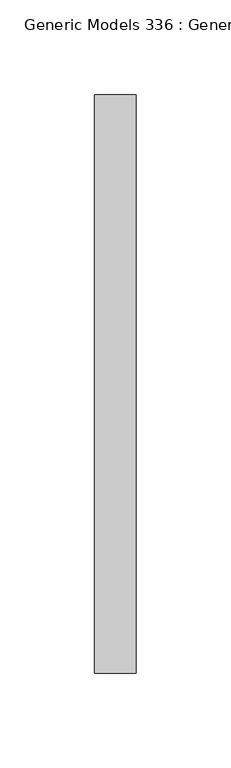
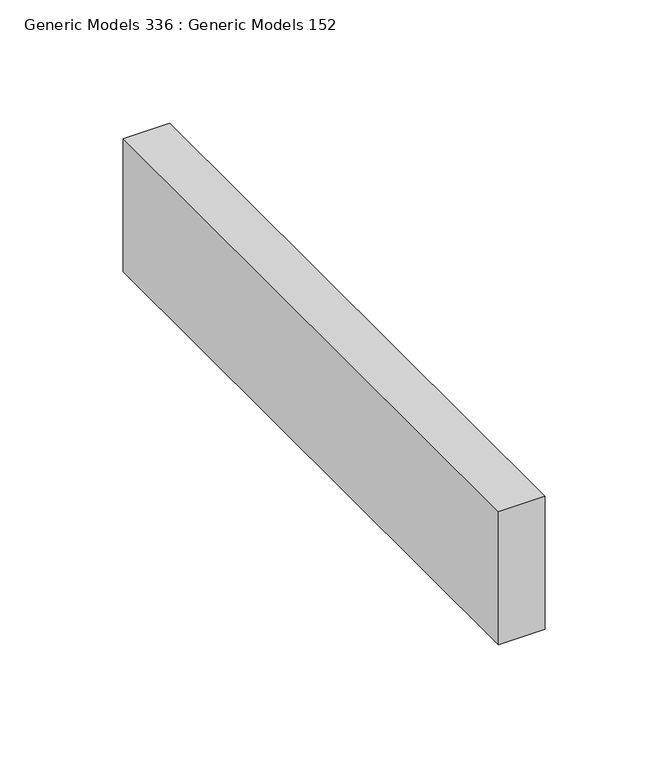
"""IFC4 building model written with IfcOpenShell, lengths in millimetres: proxy geometry, Generic Models 336 : Generic Models 152."""

import ifcopenshell
import ifcopenshell.guid

model = None  # the IFC model being written
_history = None  # IfcOwnerHistory: only IFC2X3 demands one
_inside = {}  # id of a spatial element -> (the spatial element, [elements in it])
_under = {}  # id of a project, library or spatial element -> (it, [spatial elements below it])
_declared = {}  # id of a project -> (the project, [libraries it declares])
_typed = {}  # id of a type object -> (the type object, [elements of that type])
_made_of = {}  # id of a material, layer set ... -> (it, [elements and type objects made of it])


def new_model(schema):
    """Start an empty IFC model of exactly this schema.

    Asked for "IFC4X3", IfcOpenShell would pick the latest addendum, in which some entities
    have other attributes; the version numbers below select the first issue.
    IFC2X3 requires an IfcOwnerHistory on every rooted entity: one is made here for all.
    """
    global model, _history
    if schema == "IFC4X3":
        model = ifcopenshell.file(schema_version=(4, 3, 0, 0))
    else:
        model = ifcopenshell.file(schema=schema)
    _inside.clear()
    _under.clear()
    _declared.clear()
    _typed.clear()
    _made_of.clear()
    _history = None
    if model.schema == "IFC2X3":
        org = make("IfcOrganization", Name="unknown")
        user = make(
            "IfcPersonAndOrganization",
            ThePerson=make("IfcPerson", FamilyName="unknown"),
            TheOrganization=org,
        )
        app = make(
            "IfcApplication",
            ApplicationDeveloper=org,
            Version="unknown",
            ApplicationFullName="unknown",
            ApplicationIdentifier="unknown",
        )
        _history = make(
            "IfcOwnerHistory",
            OwningUser=user,
            OwningApplication=app,
            ChangeAction="ADDED",
            CreationDate=0,
        )
    return model


def make(cls, **values):
    """One entity of the class cls with the attributes given. An attribute that is None is left unset."""
    return model.create_entity(
        cls, **{name: value for name, value in values.items() if value is not None}
    )


def rooted(cls, **values):
    """An entity with a GlobalId (a new one), such as an element, a storey or a relation."""
    return make(cls, GlobalId=ifcopenshell.guid.new(), OwnerHistory=_history, **values)


def si_unit(unit_type, name, prefix=None):
    """IfcSIUnit, for example si_unit("LENGTHUNIT", "METRE", prefix="MILLI")."""
    return make("IfcSIUnit", UnitType=unit_type, Prefix=prefix, Name=name)


def assignment(units):
    """IfcUnitAssignment: the units of a project."""
    return None if units is None else make("IfcUnitAssignment", Units=units)


def point(xyz):
    """IfcCartesianPoint."""
    return None if xyz is None else make("IfcCartesianPoint", Coordinates=xyz)


def direction(xyz):
    """IfcDirection."""
    return None if xyz is None else make("IfcDirection", DirectionRatios=xyz)


def frame(location, z_axis=None, x_axis=None):
    """IfcAxis2Placement3D, a coordinate frame: its origin and axes. An axis left out is left unset."""
    return make(
        "IfcAxis2Placement3D",
        Location=point(location),
        Axis=direction(z_axis),
        RefDirection=direction(x_axis),
    )


def origin():
    """The frame at (0, 0, 0) with its axes left unset."""
    return frame((0.0, 0.0, 0.0))


def place(relative_to, where):
    """IfcLocalPlacement: puts the frame where relative to a parent placement (None: the world)."""
    return make(
        "IfcLocalPlacement", PlacementRelTo=relative_to, RelativePlacement=where
    )


def context(
    kind, dimensions, precision=None, world=None, true_north=None, identifier=None
):
    """IfcGeometricRepresentationContext, for example the 3D "Model" context."""
    return make(
        "IfcGeometricRepresentationContext",
        ContextIdentifier=identifier,
        ContextType=kind,
        CoordinateSpaceDimension=dimensions,
        Precision=precision,
        WorldCoordinateSystem=world,
        TrueNorth=true_north,
    )


def project(units=None, contexts=None):
    """IfcProject with its units and contexts."""
    return rooted(
        "IfcProject",
        Name="project",
        RepresentationContexts=contexts,
        UnitsInContext=assignment(units),
    )


def spatial(cls, under=None, at=None, **own):
    """A site, building, storey or space (cls), placed at a placement, below another one or the project."""
    s = rooted(cls, ObjectPlacement=at, **own)
    if under is not None:
        _under.setdefault(under.id(), (under, []))[1].append(s)
    return s


def polyline(points):
    """IfcPolyline through the points."""
    return make("IfcPolyline", Points=[point(p) for p in points])


def outline(outer, holes=None, kind="AREA"):
    """IfcArbitraryClosedProfileDef: a profile drawn as a closed curve; with holes, ...WithVoids."""
    if holes is None:
        return make("IfcArbitraryClosedProfileDef", ProfileType=kind, OuterCurve=outer)
    return make(
        "IfcArbitraryProfileDefWithVoids",
        ProfileType=kind,
        OuterCurve=outer,
        InnerCurves=holes,
    )


def extrude(swept, where, along, depth):
    """IfcExtrudedAreaSolid: the profile swept, set in the frame where, extruded along a direction by depth."""
    return make(
        "IfcExtrudedAreaSolid",
        SweptArea=swept,
        Position=where,
        ExtrudedDirection=direction(along),
        Depth=depth,
    )


def shape(context_of_items, identifier, shape_type, items):
    """IfcShapeRepresentation: the items that make up one representation, for example the "Body"."""
    return make(
        "IfcShapeRepresentation",
        ContextOfItems=context_of_items,
        RepresentationIdentifier=identifier,
        RepresentationType=shape_type,
        Items=items,
    )


def source(mapping_origin, context_of_items, identifier, shape_type, items):
    """IfcRepresentationMap: a shape defined once, which mapped items show again and again."""
    return make(
        "IfcRepresentationMap",
        MappingOrigin=mapping_origin,
        MappedRepresentation=shape(context_of_items, identifier, shape_type, items),
    )


def transform(
    local_origin,
    x_axis=None,
    y_axis=None,
    z_axis=None,
    scale=None,
    scale2=None,
    scale3=None,
    uniform=True,
):
    """IfcCartesianTransformationOperator3D, or its non-uniform kind. x_axis, y_axis, z_axis: its Axis1, 2, 3."""
    if uniform:
        return make(
            "IfcCartesianTransformationOperator3D",
            Axis1=direction(x_axis),
            Axis2=direction(y_axis),
            LocalOrigin=point(local_origin),
            Scale=scale,
            Axis3=direction(z_axis),
        )
    return make(
        "IfcCartesianTransformationOperator3DnonUniform",
        Axis1=direction(x_axis),
        Axis2=direction(y_axis),
        LocalOrigin=point(local_origin),
        Scale=scale,
        Axis3=direction(z_axis),
        Scale2=scale2,
        Scale3=scale3,
    )


def mapped(mapping_source, mapping_target):
    """IfcMappedItem: shows the shape of a source again, moved by a transform."""
    return make(
        "IfcMappedItem", MappingSource=mapping_source, MappingTarget=mapping_target
    )


def made_of(thing, what):
    """Note that an element or type object is made of a material, layer set ...; save() writes the relation."""
    if what is not None:
        _made_of.setdefault(what.id(), (what, []))[1].append(thing)
    return thing


def element(
    cls,
    number,
    at=None,
    inside=None,
    cuts=None,
    type_object=None,
    material=None,
    context=None,
    identifier="Body",
    shape_type=None,
    held_by="IfcProductDefinitionShape",
    body=None,
    shapes=None,
    **own,
):
    """One element of the class cls, such as IfcWall. Its Tag is "e" and its number.

    at: its placement. inside: the storey or other place that contains it. cuts: it is an
    opening in that element (IfcRelVoidsElement). A single representation is given by context,
    identifier, shape_type and body (its items); several are given by shapes. held_by: the class
    of the entity that holds the representations. save() writes the other relations.
    """
    e = rooted(cls, Tag="e%d" % number, ObjectPlacement=at, **own)
    if body is not None:
        shapes = [shape(context, identifier, shape_type, body)]
    if shapes is not None:
        e.Representation = make(held_by, Representations=shapes)
    if inside is not None:
        _inside.setdefault(inside.id(), (inside, []))[1].append(e)
    if cuts is not None:
        rooted(
            "IfcRelVoidsElement", RelatingBuildingElement=cuts, RelatedOpeningElement=e
        )
    if type_object is not None:
        _typed.setdefault(type_object.id(), (type_object, []))[1].append(e)
    return made_of(e, material)


def aggregate(whole, parts):
    """IfcRelAggregates: a whole, such as a stair, and the parts it consists of."""
    return rooted("IfcRelAggregates", RelatingObject=whole, RelatedObjects=parts)


def save(model, path):
    """Write the relations noted so far, then the file.

    IfcRelAggregates (storeys below a building ...), IfcRelContainedInSpatialStructure (elements
    in a storey), IfcRelDefinesByType, IfcRelAssociatesMaterial and IfcRelDeclares: one each for
    every whole, place, type object, material and project.
    """
    for whole, parts in _under.values():
        aggregate(whole, parts)
    for where, things in _inside.values():
        rooted(
            "IfcRelContainedInSpatialStructure",
            RelatedElements=things,
            RelatingStructure=where,
        )
    for kind, things in _typed.values():
        rooted("IfcRelDefinesByType", RelatedObjects=things, RelatingType=kind)
    for what, things in _made_of.values():
        rooted("IfcRelAssociatesMaterial", RelatedObjects=things, RelatingMaterial=what)
    for by, libraries in _declared.values():
        rooted("IfcRelDeclares", RelatingContext=by, RelatedDefinitions=libraries)
    model.write(path)


def generic_models_336_generic_models_152_2bdf3ea2(model_context):
    return source(origin(), model_context, "Body", "SweptSolid", [
        extrude(outline(polyline([(4826.1808084, 704.5309662), (4848.0773272, 704.5309662), (4848.0773272, 399.7309662), (4826.1808084, 399.7309662), (4826.1808084, 704.5309662)])), frame((0.0, 0.0, 126190.7673937), z_axis=(0.0, 0.0, 1.0), x_axis=(1.0, 0.0, 0.0)), (0.0, 0.0, 1.0), 66.0286063),
    ])


if __name__ == "__main__":
    model = new_model("IFC4")
    model_context = context("Model", 3, world=origin())
    ifc_project = project(units=[si_unit("LENGTHUNIT", "METRE", prefix="MILLI")], contexts=[model_context])
    site = spatial("IfcSite", under=ifc_project)
    building = spatial("IfcBuilding", under=site)
    placement = place(None, origin())
    generic_models_336_generic_models_152_shape = generic_models_336_generic_models_152_2bdf3ea2(model_context)
    element("IfcBuildingElementProxy", 1, Name="Generic Models 336 : Generic Models 152", ObjectType="Generic Models 336 : Generic Models 152", at=placement, inside=building, context=model_context, shape_type="MappedRepresentation", body=[
        mapped(generic_models_336_generic_models_152_shape, transform((0.0, 0.0, 0.0), x_axis=(1.0, 0.0, 0.0), y_axis=(0.0, 1.0, 0.0), z_axis=(0.0, 0.0, 1.0))),
    ])
    save(model, "model.ifc")

# Revit data of these elements
# Element 1 (IfcBuildingElementProxy, "Generic Models 336 : Generic Models 152")
#   Materials on its faces: "_BLOCKING AS REQUIRED"
# Materials
#   "_BLOCKING AS REQUIRED": class "Generic", colour RGB 177 130 114, transparency 0, Cost = 0
